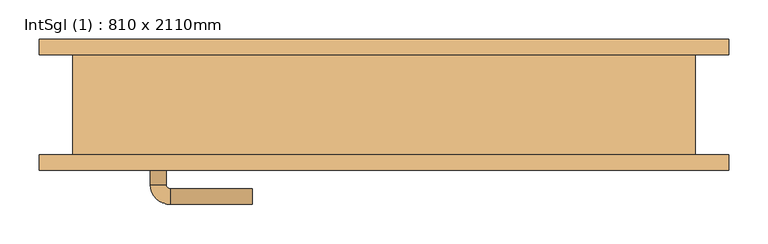
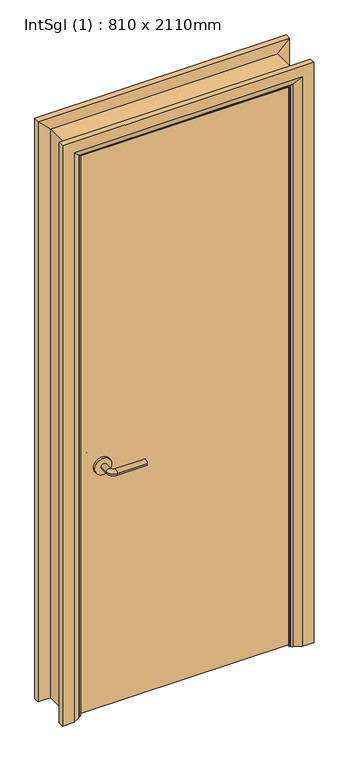
"""IFC4 building model written with IfcOpenShell, lengths in millimetres: door geometry, IntSgl (1) : 810 x 2110mm."""

from ifc_helpers import new_model, si_unit, point, frame, frame_2d, origin, place, context, project, spatial, polyline, circle_curve, ellipse_curve, trimmed, segment, composite_curve, outline, extrude, faceted_brep, source, transform, mapped, element, save
from ifc_brep_helpers import plane_surface, cylinder_surface, revolved_surface, advanced_brep


def intsgl_1_810_x_2110mm_198b6b43(model_context):
    return source(origin(), model_context, "Body", "SolidModel", [
        advanced_brep(
        [(-298.0, -17.75, 900.0), (-278.0, -17.75, 900.0), (-298.0, 12.25, 900.0), (-278.0, 12.25, 900.0), (-273.0, 17.25, 900.0), (-273.0, 37.25, 900.0), (-168.0, 37.25, 900.0), (-168.0, 17.25, 900.0)],
        [
            (0, 1, circle_curve(frame((-288.0, -17.75, 900.0), z_axis=(0.0, -1.0, 0.0), x_axis=(1.0, 0.0, 0.0)), 10.0)),
            (1, 0, circle_curve(frame((-288.0, -17.75, 900.0), z_axis=(0.0, -1.0, 0.0), x_axis=(1.0, 0.0, 0.0)), 10.0)),
            (0, 2),
            (2, 3, circle_curve(frame((-288.0, 12.25, 900.0), z_axis=(0.0, -1.0, 0.0), x_axis=(1.0, 0.0, 0.0)), 10.0)),
            (3, 1),
            (3, 2, circle_curve(frame((-288.0, 12.25, 900.0), z_axis=(0.0, -1.0, 0.0), x_axis=(1.0, 0.0, 0.0)), 10.0)),
            (4, 3, circle_curve(frame((-273.0, 12.25, 900.0), z_axis=(0.0, 0.0, 1.0), x_axis=(-1.0, 0.0, 0.0)), 5.0)),
            (2, 5, circle_curve(frame((-273.0, 12.25, 900.0), z_axis=(0.0, 0.0, -1.0), x_axis=(-1.0, 0.0, 0.0)), 25.0)),
            (5, 4, circle_curve(frame((-273.0, 27.25, 900.0), z_axis=(-1.0, 0.0, 0.0), x_axis=(0.0, -1.0, 0.0)), 10.0)),
            (4, 5, circle_curve(frame((-273.0, 27.25, 900.0), z_axis=(-1.0, 0.0, 0.0), x_axis=(0.0, -1.0, 0.0)), 10.0)),
            (6, 7, circle_curve(frame((-168.0, 27.25, 900.0), z_axis=(1.0, 0.0, 0.0), x_axis=(0.0, -1.0, 0.0)), 10.0)),
            (7, 6, circle_curve(frame((-168.0, 27.25, 900.0), z_axis=(1.0, 0.0, 0.0), x_axis=(0.0, -1.0, 0.0)), 10.0)),
            (5, 6),
            (7, 4),
        ],
        [
            plane_surface(frame((-288.0, -17.75, 900.0), z_axis=(0.0, -1.0, 0.0), x_axis=(0.0, 0.0, 1.0))),
            cylinder_surface(frame((-288.0, -17.75, 900.0), z_axis=(0.0, -1.0, 0.0), x_axis=(1.0, 0.0, 0.0)), 10.0),
            revolved_surface(trimmed(ellipse_curve(frame((-288.0, 12.25, 900.0), z_axis=(0.0, -1.0, 0.0), x_axis=(1.0, 0.0, 0.0)), 10.0, 10.0), [point((-298.0, 12.25, 900.0))], [point((-278.0, 12.25, 900.0))], True, "CARTESIAN"), (-273.0, 12.25, 900.0), (0.0, 0.0, -1.0)),
            revolved_surface(trimmed(ellipse_curve(frame((-288.0, 12.25, 900.0), z_axis=(0.0, -1.0, 0.0), x_axis=(1.0, 0.0, 0.0)), 10.0, 10.0), [point((-278.0, 12.25, 900.0))], [point((-298.0, 12.25, 900.0))], True, "CARTESIAN"), (-273.0, 12.25, 900.0), (0.0, 0.0, -1.0)),
            plane_surface(frame((-168.0, 27.25, 900.0), z_axis=(1.0, 0.0, 0.0), x_axis=(0.0, 0.0, 1.0))),
            cylinder_surface(frame((-273.0, 27.25, 900.0), z_axis=(-1.0, 0.0, 0.0), x_axis=(0.0, -1.0, 0.0)), 10.0),
        ],
        [
            (0, [[1, 2]]),
            (1, [[-1, 3, 4, 5]]),
            (1, [[-2, -5, 6, -3]]),
            (2, [[7, -4, 8, 9]]),
            (3, [[-8, -6, -7, 10]]),
            (4, [[11, 12]]),
            (5, [[-9, 13, -12, 14]]),
            (5, [[-10, -14, -11, -13]]),
        ],
    ),
        extrude(outline(composite_curve([segment(trimmed(circle_curve(frame_2d((900.0, -290.5)), 30.0), [point((900.0, -320.5))], [point((900.0, -260.5))], False, "CARTESIAN"), True, "CONTINUOUS"), segment(trimmed(circle_curve(frame_2d((900.0, -290.5)), 30.0), [point((900.0, -260.5))], [point((900.0, -320.5))], False, "CARTESIAN"), True, "CONTINUOUS")], self_intersect=False)), frame((0.0, -25.75, 0.0), z_axis=(0.0, 1.0, 0.0), x_axis=(0.0, 0.0, 1.0)), (0.0, 0.0, 1.0), 8.0),
        advanced_brep(
        [(-298.0, -71.75, 900.0), (-278.0, -71.75, 900.0), (-278.0, -101.75, 900.0), (-298.0, -101.75, 900.0), (-273.0, -106.75, 900.0), (-273.0, -126.75, 900.0), (-168.0, -126.75, 900.0), (-168.0, -106.75, 900.0)],
        [
            (0, 1, circle_curve(frame((-288.0, -71.75, 900.0), z_axis=(0.0, 1.0, 0.0), x_axis=(1.0, 0.0, 0.0)), 10.0)),
            (1, 0, circle_curve(frame((-288.0, -71.75, 900.0), z_axis=(0.0, 1.0, 0.0), x_axis=(1.0, 0.0, 0.0)), 10.0)),
            (1, 2),
            (2, 3, circle_curve(frame((-288.0, -101.75, 900.0), z_axis=(0.0, 1.0, 0.0), x_axis=(1.0, 0.0, 0.0)), 10.0)),
            (3, 0),
            (3, 2, circle_curve(frame((-288.0, -101.75, 900.0), z_axis=(0.0, 1.0, 0.0), x_axis=(1.0, 0.0, 0.0)), 10.0)),
            (4, 5, circle_curve(frame((-273.0, -116.75, 900.0), z_axis=(-1.0, 0.0, 0.0), x_axis=(0.0, 1.0, 0.0)), 10.0)),
            (5, 3, circle_curve(frame((-273.0, -101.75, 900.0), z_axis=(0.0, 0.0, -1.0), x_axis=(-1.0, 0.0, 0.0)), 25.0)),
            (2, 4, circle_curve(frame((-273.0, -101.75, 900.0), z_axis=(0.0, 0.0, 1.0), x_axis=(-1.0, 0.0, 0.0)), 5.0)),
            (5, 4, circle_curve(frame((-273.0, -116.75, 900.0), z_axis=(-1.0, 0.0, 0.0), x_axis=(0.0, 1.0, 0.0)), 10.0)),
            (6, 7, circle_curve(frame((-168.0, -116.75, 900.0), z_axis=(1.0, 0.0, 0.0), x_axis=(0.0, 1.0, 0.0)), 10.0)),
            (7, 6, circle_curve(frame((-168.0, -116.75, 900.0), z_axis=(1.0, 0.0, 0.0), x_axis=(0.0, 1.0, 0.0)), 10.0)),
            (4, 7),
            (6, 5),
        ],
        [
            plane_surface(frame((-288.0, -71.75, 900.0), z_axis=(0.0, 1.0, 0.0), x_axis=(0.0, 0.0, 1.0))),
            cylinder_surface(frame((-288.0, -71.75, 900.0), z_axis=(0.0, 1.0, 0.0), x_axis=(1.0, 0.0, 0.0)), 10.0),
            revolved_surface(trimmed(ellipse_curve(frame((-288.0, -101.75, 900.0), z_axis=(0.0, -1.0, 0.0), x_axis=(1.0, 0.0, 0.0)), 10.0, 10.0), [point((-298.0, -101.75, 900.0))], [point((-278.0, -101.75, 900.0))], True, "CARTESIAN"), (-273.0, -101.75, 900.0), (0.0, 0.0, -1.0)),
            revolved_surface(trimmed(ellipse_curve(frame((-288.0, -101.75, 900.0), z_axis=(0.0, -1.0, 0.0), x_axis=(1.0, 0.0, 0.0)), 10.0, 10.0), [point((-278.0, -101.75, 900.0))], [point((-298.0, -101.75, 900.0))], True, "CARTESIAN"), (-273.0, -101.75, 900.0), (0.0, 0.0, -1.0)),
            plane_surface(frame((-168.0, -116.75, 900.0), z_axis=(1.0, 0.0, 0.0), x_axis=(0.0, 0.0, 1.0))),
            cylinder_surface(frame((-273.0, -116.75, 900.0), z_axis=(-1.0, 0.0, 0.0), x_axis=(0.0, 1.0, 0.0)), 10.0),
        ],
        [
            (0, [[1, 2]]),
            (1, [[3, 4, 5, -2]]),
            (1, [[-5, 6, -3, -1]]),
            (2, [[7, 8, -4, 9]]),
            (3, [[10, -9, -6, -8]]),
            (4, [[11, 12]]),
            (5, [[13, -11, 14, -7]]),
            (5, [[-14, -12, -13, -10]]),
        ],
    ),
        extrude(outline(composite_curve([segment(trimmed(circle_curve(frame_2d((900.0, -290.5)), 30.0), [point((900.0, -320.5))], [point((900.0, -260.5))], False, "CARTESIAN"), True, "CONTINUOUS"), segment(trimmed(circle_curve(frame_2d((900.0, -290.5)), 30.0), [point((900.0, -260.5))], [point((900.0, -320.5))], False, "CARTESIAN"), True, "CONTINUOUS")], self_intersect=False)), frame((0.0, -71.75, 0.0), z_axis=(0.0, 1.0, 0.0), x_axis=(0.0, 0.0, 1.0)), (0.0, 0.0, 1.0), 8.0),
        extrude(outline(polyline([(363.0, -25.75), (363.0, -63.75), (-363.0, -63.75), (-363.0, -25.75), (363.0, -25.75)])), frame((0.0, 0.0, 8.0), z_axis=(0.0, 0.0, 1.0), x_axis=(1.0, 0.0, 0.0)), (0.0, 0.0, 1.0), 2060.0),
        advanced_brep(
        [(440.0, -83.75, 0.0), (400.0, -83.75, 0.0), (374.0, -69.75, 0.0), (370.0, -63.75, 0.0), (440.0, -63.75, 0.0), (440.0, -63.75, 2145.0), (440.0, -83.75, 2145.0), (370.0, -63.75, 2075.0), (-370.0, -63.75, 2075.0), (-370.0, -63.75, 0.0), (-440.0, -63.75, 0.0), (-440.0, -63.75, 2145.0), (374.0, -69.75, 2079.0), (400.0, -83.75, 2105.0), (-440.0, -83.75, 2145.0), (-440.0, -83.75, 0.0), (-400.0, -83.75, 0.0), (-400.0, -83.75, 2105.0), (-374.0, -69.75, 2079.0), (-374.0, -69.75, 0.0)],
        [
            (0, 1),
            (1, 2),
            (2, 3, circle_curve(frame((378.0, -62.75, 0.0), z_axis=(0.0, 0.0, -1.0), x_axis=(1.0, 0.0, 0.0)), 8.0622577)),
            (3, 4),
            (4, 0),
            (4, 5),
            (5, 6),
            (6, 0),
            (3, 7),
            (7, 8),
            (8, 9),
            (9, 10),
            (10, 11),
            (11, 5),
            (2, 12),
            (12, 7, ellipse_curve(frame((378.0, -62.75, 2083.0), z_axis=(0.7071067811865475, 0.0, -0.7071067811865475), x_axis=(-0.7071067811865474, 0.0, -0.7071067811865476)), 11.4017543, 8.0622577)),
            (1, 13),
            (13, 12),
            (6, 14),
            (14, 15),
            (15, 16),
            (16, 17),
            (17, 13),
            (11, 14),
            (12, 18),
            (18, 8, ellipse_curve(frame((-378.0, -62.75, 2083.0), z_axis=(0.7071067811865475, 0.0, 0.7071067811865475), x_axis=(0.7071067811865476, 0.0, -0.7071067811865474)), 11.4017543, 8.0622577)),
            (17, 18),
            (15, 10),
            (9, 19, circle_curve(frame((-378.0, -62.75, 0.0), z_axis=(0.0, 0.0, -1.0), x_axis=(-1.0, 0.0, 0.0)), 8.0622577)),
            (19, 16),
            (18, 19),
        ],
        [
            plane_surface(frame((370.0, -63.75, 0.0), z_axis=(0.0, 0.0, -1.0), x_axis=(0.0, 1.0, 0.0))),
            plane_surface(frame((440.0, -83.75, 0.0), z_axis=(1.0, 0.0, 0.0), x_axis=(0.0, 0.0, 1.0))),
            plane_surface(frame((440.0, -63.75, 0.0), z_axis=(0.0, 1.0, 0.0), x_axis=(0.0, 0.0, 1.0))),
            cylinder_surface(frame((378.0, -62.75, 0.0), z_axis=(0.0, 0.0, -1.0), x_axis=(1.0, 0.0, 0.0)), 8.0622577),
            plane_surface(frame((374.0, -69.75, 0.0), z_axis=(-0.4740998230350126, -0.880471099922178, 0.0), x_axis=(0.0, 0.0, 1.0))),
            plane_surface(frame((400.0, -83.75, 0.0), z_axis=(0.0, -1.0, 0.0), x_axis=(0.0, 0.0, 1.0))),
            plane_surface(frame((440.0, -83.75, 2145.0), z_axis=(0.0, 0.0, 1.0), x_axis=(-1.0, 0.0, 0.0))),
            cylinder_surface(frame((370.0, -62.75, 2083.0), z_axis=(1.0, 0.0, 0.0), x_axis=(0.0, 0.0, 1.0)), 8.0622577),
            plane_surface(frame((374.0, -69.75, 2079.0), z_axis=(0.0, -0.8804710999221764, -0.4740998230350154), x_axis=(-1.0, 0.0, 0.0))),
            plane_surface(frame((-370.0, -63.75, 0.0), z_axis=(0.0, 0.0, -1.0), x_axis=(0.0, 1.0, 0.0))),
            plane_surface(frame((-440.0, -83.75, 2145.0), z_axis=(-1.0, 0.0, 0.0), x_axis=(0.0, 0.0, -1.0))),
            cylinder_surface(frame((-378.0, -62.75, 2075.0), z_axis=(0.0, 0.0, 1.0), x_axis=(-1.0, 0.0, 0.0)), 8.0622577),
            plane_surface(frame((-374.0, -69.75, 2079.0), z_axis=(0.47409982303501824, -0.8804710999221749, 0.0), x_axis=(0.0, 0.0, -1.0))),
        ],
        [
            (0, [[1, 2, 3, 4, 5]]),
            (1, [[6, 7, 8, -5]]),
            (2, [[9, 10, 11, 12, 13, 14, -6, -4]]),
            (3, [[15, 16, -9, -3]]),
            (4, [[17, 18, -15, -2]]),
            (5, [[-8, 19, 20, 21, 22, 23, -17, -1]]),
            (6, [[-14, 24, -19, -7]]),
            (7, [[25, 26, -10, -16]]),
            (8, [[-23, 27, -25, -18]]),
            (9, [[28, -12, 29, 30, -21]]),
            (10, [[-13, -28, -20, -24]]),
            (11, [[31, -29, -11, -26]]),
            (12, [[-22, -30, -31, -27]]),
        ],
    ),
        extrude(outline(polyline([(0.0, -346.0), (2051.0, -346.0), (2051.0, 346.0), (0.0, 346.0), (0.0, 365.0), (2070.0, 365.0), (2070.0, -365.0), (0.0, -365.0), (0.0, -346.0)])), frame((0.0, -23.75, 0.0), z_axis=(0.0, 1.0, 0.0), x_axis=(0.0, 0.0, 1.0)), (0.0, 0.0, 1.0), 32.0),
        advanced_brep(
        [(-440.0, 83.75, 0.0), (-400.0, 83.75, 0.0), (-374.0, 69.75, 0.0), (-370.0, 63.75, 0.0), (-440.0, 63.75, 0.0), (-440.0, 63.75, 2145.0), (-440.0, 83.75, 2145.0), (-370.0, 63.75, 2075.0), (-374.0, 69.75, 2079.0), (-400.0, 83.75, 2105.0), (440.0, 63.75, 2145.0), (440.0, 83.75, 2145.0), (370.0, 63.75, 2075.0), (374.0, 69.75, 2079.0), (400.0, 83.75, 2105.0), (440.0, 83.75, 0.0), (440.0, 63.75, 0.0), (370.0, 63.75, 0.0), (374.0, 69.75, 0.0), (400.0, 83.75, 0.0)],
        [
            (0, 1),
            (1, 2),
            (2, 3, circle_curve(frame((-378.0, 62.75, 0.0), z_axis=(0.0, 0.0, -1.0), x_axis=(-1.0, 0.0, 0.0)), 8.0622577)),
            (3, 4),
            (4, 0),
            (4, 5),
            (5, 6),
            (6, 0),
            (3, 7),
            (7, 5),
            (2, 8),
            (8, 7, ellipse_curve(frame((-378.0, 62.75, 2083.0), z_axis=(-0.7071067811865475, 0.0, -0.7071067811865475), x_axis=(0.7071067811865474, 0.0, -0.7071067811865476)), 11.4017543, 8.0622577)),
            (1, 9),
            (9, 8),
            (6, 9),
            (5, 10),
            (10, 11),
            (11, 6),
            (7, 12),
            (12, 10),
            (8, 13),
            (13, 12, ellipse_curve(frame((378.0, 62.75, 2083.0), z_axis=(-0.7071067811865475, 0.0, 0.7071067811865475), x_axis=(-0.7071067811865476, 0.0, -0.7071067811865474)), 11.4017543, 8.0622577)),
            (9, 14),
            (14, 13),
            (11, 14),
            (15, 16),
            (16, 17),
            (17, 18, circle_curve(frame((378.0, 62.75, 0.0), z_axis=(0.0, 0.0, -1.0), x_axis=(1.0, 0.0, 0.0)), 8.0622577)),
            (18, 19),
            (19, 15),
            (10, 16),
            (15, 11),
            (12, 17),
            (13, 18),
            (14, 19),
        ],
        [
            plane_surface(frame((-370.0, 136.5510989, 0.0), z_axis=(0.0, 0.0, -1.0), x_axis=(1.0, 0.0, 0.0))),
            plane_surface(frame((-440.0, 83.75, 0.0), z_axis=(-1.0, 0.0, 0.0), x_axis=(0.0, 0.0, 1.0))),
            plane_surface(frame((-440.0, 63.75, 0.0), z_axis=(0.0, -1.0, 0.0), x_axis=(0.0, 0.0, 1.0))),
            cylinder_surface(frame((-378.0, 62.75, 0.0), z_axis=(0.0, 0.0, -1.0), x_axis=(-1.0, 0.0, 0.0)), 8.0622577),
            plane_surface(frame((-374.0, 69.75, 0.0), z_axis=(0.4740998230350183, 0.8804710999221749, 0.0), x_axis=(0.0, 0.0, 1.0))),
            plane_surface(frame((-400.0, 83.75, 0.0), z_axis=(0.0, 1.0, 0.0), x_axis=(0.0, 0.0, 1.0))),
            plane_surface(frame((-440.0, 83.75, 2145.0), z_axis=(0.0, 0.0, 1.0), x_axis=(1.0, 0.0, 0.0))),
            plane_surface(frame((-440.0, 63.75, 2145.0), z_axis=(0.0, -1.0, 0.0), x_axis=(1.0, 0.0, 0.0))),
            cylinder_surface(frame((-370.0, 62.75, 2083.0), z_axis=(-1.0, 0.0, 0.0), x_axis=(0.0, 0.0, 1.0)), 8.0622577),
            plane_surface(frame((-374.0, 69.75, 2079.0), z_axis=(0.0, 0.8804710999221749, -0.4740998230350183), x_axis=(1.0, 0.0, 0.0))),
            plane_surface(frame((-400.0, 83.75, 2105.0), z_axis=(0.0, 1.0, 0.0), x_axis=(1.0, 0.0, 0.0))),
            plane_surface(frame((370.0, 136.5510989, 0.0), z_axis=(0.0, 0.0, -1.0), x_axis=(-1.0, 0.0, 0.0))),
            plane_surface(frame((440.0, 83.75, 2145.0), z_axis=(1.0, 0.0, 0.0), x_axis=(0.0, 0.0, -1.0))),
            plane_surface(frame((440.0, 63.75, 2145.0), z_axis=(0.0, -1.0, 0.0), x_axis=(0.0, 0.0, -1.0))),
            cylinder_surface(frame((378.0, 62.75, 2075.0), z_axis=(0.0, 0.0, 1.0), x_axis=(1.0, 0.0, 0.0)), 8.0622577),
            plane_surface(frame((374.0, 69.75, 2079.0), z_axis=(-0.4740998230350183, 0.8804710999221749, 0.0), x_axis=(0.0, 0.0, -1.0))),
            plane_surface(frame((400.0, 83.75, 2105.0), z_axis=(0.0, 1.0, 0.0), x_axis=(0.0, 0.0, -1.0))),
        ],
        [
            (0, [[1, 2, 3, 4, 5]]),
            (1, [[6, 7, 8, -5]]),
            (2, [[9, 10, -6, -4]]),
            (3, [[11, 12, -9, -3]]),
            (4, [[13, 14, -11, -2]]),
            (5, [[-8, 15, -13, -1]]),
            (6, [[16, 17, 18, -7]]),
            (7, [[19, 20, -16, -10]]),
            (8, [[21, 22, -19, -12]]),
            (9, [[23, 24, -21, -14]]),
            (10, [[-18, 25, -23, -15]]),
            (11, [[26, 27, 28, 29, 30]]),
            (12, [[31, -26, 32, -17]]),
            (13, [[33, -27, -31, -20]]),
            (14, [[34, -28, -33, -22]]),
            (15, [[35, -29, -34, -24]]),
            (16, [[-32, -30, -35, -25]]),
        ],
    ),
        faceted_brep([(-365.0, -63.75, 0.0), (-397.0, -63.75, 0.0), (-397.0, 63.75, 0.0), (-365.0, 63.75, 0.0), (-365.0, 63.75, 2070.0), (-365.0, -63.75, 2070.0), (-397.0, 63.75, 2102.0), (-397.0, -63.75, 2102.0), (365.0, 63.75, 2070.0), (365.0, -63.75, 2070.0), (397.0, 63.75, 2102.0), (397.0, -63.75, 2102.0), (365.0, -63.75, 0.0), (365.0, 63.75, 0.0), (397.0, 63.75, 0.0), (397.0, -63.75, 0.0)], [[[0, 1, 2, 3]], [[3, 4, 5, 0]], [[2, 6, 4, 3]], [[1, 7, 6, 2]], [[0, 5, 7, 1]], [[4, 8, 9, 5]], [[6, 10, 8, 4]], [[7, 11, 10, 6]], [[5, 9, 11, 7]], [[12, 13, 14, 15]], [[8, 13, 12, 9]], [[10, 14, 13, 8]], [[11, 15, 14, 10]], [[9, 12, 15, 11]]]),
    ])


if __name__ == "__main__":
    model = new_model("IFC4")
    model_context = context("Model", 3, world=origin())
    ifc_project = project(units=[si_unit("LENGTHUNIT", "METRE", prefix="MILLI")], contexts=[model_context])
    site = spatial("IfcSite", under=ifc_project)
    building = spatial("IfcBuilding", under=site)
    placement = place(None, origin())
    intsgl_1_810_x_2110mm_shape = intsgl_1_810_x_2110mm_198b6b43(model_context)
    element("IfcDoor", 1, ObjectType="IntSgl (1) : 810 x 2110mm", at=placement, inside=building, context=model_context, shape_type="MappedRepresentation", body=[
        mapped(intsgl_1_810_x_2110mm_shape, transform((0.0, 0.0, 0.0), x_axis=(1.0, 0.0, 0.0), y_axis=(0.0, 1.0, 0.0), z_axis=(0.0, 0.0, 1.0))),
    ])
    save(model, "model.ifc")

# Revit data of these elements
# Type "IntSgl (1) : 810 x 2110mm"
#   Construction Type Id = "MDOOR"
#   Analytic Construction = "Metal"
#   Type Mark = "42"
#   Type Comments = "Internal Single"
#   Operation = "SingleSwingRight"
#   Manufacturer = "Revit"
#   Keynote = "L20"
#   Description = "Internal Single Door"
#   Visual Light Transmittance = 0
#   Solar Heat Gain Coefficient = 0
#   Heat Transfer Coefficient (U) = 3.7021 W/(m²·K)
#   UnderCut = 8 mm
#   Tolerance = 2 mm
#   Thickness = 38 mm
#   Structural Tolerance = 8 mm
#   StopDepth = 32 mm
#   Stop Thickness = 19 mm
#   Rough Width = 810 mm
#   Rough Height = 2110 mm
#   Height to Top Lock Rail = 1000 mm
#   Handle Z Distance = 900 mm
#   Handle X Distance = 75 mm
#   Frame Thickness = 32 mm
#   Door Panel Width = 726 mm
#   Door Panel Thickness = 38 mm
#   Door Panel Offset = 0 mm
#   Height = 2110 mm
#   Width = 810 mm
#   Door Panel Height = 2060 mm
#   Architrave Setback = 5 mm
#   Function = 0
#   Vis - Ironmongery = yes
#   Material Ironmongery = Door - Handle
#   Material Frame = Door - Frame/Mullion (1)
#   Material Door = Door - Panel
#   Material Architrave = Door - Architrave
#   Wall Closure = (empty or 0)
# Element 1 (IfcDoor, "IntSgl (1) : 810 x 2110mm")
#   Materials on its faces: "Door - Architrave", "Door - Handle", "Door - Frame/Mullion (1)", "Door - Panel"
# Materials
#   "Door - Handle": class "Miscellaneous", colour RGB 0 0 0, transparency 0, Keynote = "P21"
#   "Door - Frame/Mullion (1)": class "Wood", colour RGB 212 179 113, transparency 0, Keynote = "L20", Cost = 0
#   "Door - Panel": class "Wood", colour RGB 210 159 95, transparency 0, Keynote = "L20"
#   "Door - Architrave": class "Wood", colour RGB 154 90 5, transparency 0, Keynote = "P20"
